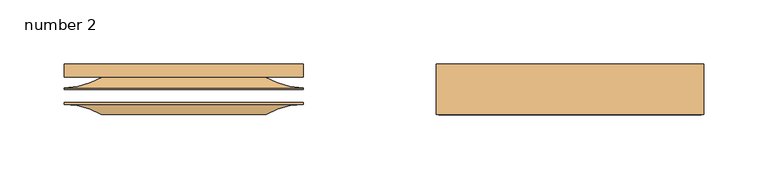
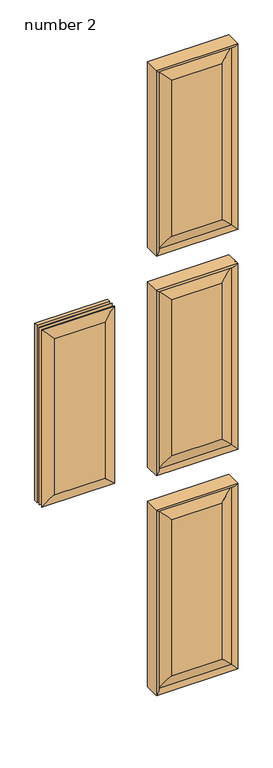
"""IFC4 building model written with IfcOpenShell, lengths in millimetres: door geometry, Door-Interior-Karona-K5660-6_Panel : number 2."""

from ifc_helpers import new_model, si_unit, frame, origin, place, context, project, spatial, polyline, ellipse_curve, source, transform, mapped, element, save
from ifc_brep_helpers import plane_surface, cylinder_surface, revolved_surface, advanced_brep


def number_2_a8c36a05(model_context):
    return source(origin(), model_context, "Body", "AdvancedBrep", [
        advanced_brep(
        [(242.8748, 54.4576, 1893.8748), (242.8748, 54.4576, 1414.4752), (57.1627, 54.4576, 1414.4752), (57.1627, 54.4576, 1893.8748), (242.8748, 34.7218, 1893.8748), (242.8748, 36.0454899, 1893.8748), (57.1627, 36.0454899, 1893.8748), (57.1627, 34.7218, 1893.8748), (57.1627, 44.5515929, 1893.8748), (242.8748, 44.5515929, 1893.8748), (57.1627, 34.7218, 1414.4752), (57.1627, 36.0454899, 1414.4752), (242.8748, 36.0454899, 1414.4752), (242.8748, 34.7218, 1414.4752), (242.8748, 44.5515929, 1414.4752), (57.1627, 44.5515929, 1414.4752), (87.1686653, 44.5515929, 1863.8688347), (212.8688347, 44.5515929, 1863.8688347), (87.1686653, 44.5515929, 1444.4811653), (212.8688347, 44.5515929, 1444.4811653)],
        [
            (0, 1),
            (1, 2),
            (2, 3),
            (3, 0),
            (4, 5),
            (5, 6),
            (6, 7),
            (7, 4),
            (3, 8),
            (8, 9),
            (9, 0),
            (10, 11),
            (11, 12),
            (12, 13),
            (13, 10),
            (1, 14),
            (14, 15),
            (15, 2),
            (9, 14),
            (12, 5),
            (4, 13),
            (6, 11),
            (10, 7),
            (15, 8),
            (16, 6, ellipse_curve(frame((55.2243315, 100.0605261, 1895.8131685), z_axis=(-0.7071067811865475, 0.0, -0.7071067811865475), x_axis=(0.7071067811865476, 0.0, -0.7071067811865474)), 90.5724254, 64.0443762)),
            (5, 17, ellipse_curve(frame((244.8131685, 100.0605261, 1895.8131685), z_axis=(0.7071067811865475, 0.0, -0.7071067811865475), x_axis=(0.7071067811865476, 0.0, 0.7071067811865474)), 90.5724254, 64.0443762)),
            (17, 16),
            (18, 11, ellipse_curve(frame((55.2243315, 100.0605261, 1412.5368315), z_axis=(0.7071067811865475, 0.0, -0.7071067811865475), x_axis=(0.7071067811865474, 0.0, 0.7071067811865476)), 90.5724254, 64.0443762)),
            (16, 18),
            (19, 12, ellipse_curve(frame((244.8131685, 100.0605261, 1412.5368315), z_axis=(0.7071067811865475, 0.0, 0.7071067811865475), x_axis=(-0.7071067811865476, 0.0, 0.7071067811865474)), 90.5724254, 64.0443762)),
            (18, 19),
            (19, 17),
        ],
        [
            plane_surface(frame((57.1627, 54.4576, 1893.8748), z_axis=(0.0, 1.0, 0.0), x_axis=(0.0, 0.0, -1.0))),
            plane_surface(frame((57.1627, 34.7218, 1893.8748), z_axis=(0.0, 0.0, 1.0), x_axis=(-1.0, 0.0, 0.0))),
            plane_surface(frame((57.1627, 34.7218, 1414.4752), z_axis=(0.0, 0.0, -1.0), x_axis=(1.0, 0.0, 0.0))),
            plane_surface(frame((242.8748, 54.4576, 1893.8748), z_axis=(1.0, 0.0, 0.0), x_axis=(0.0, 0.0, -1.0))),
            plane_surface(frame((57.1627, 34.7218, 1893.8748), z_axis=(-1.0, 0.0, 0.0), x_axis=(0.0, 0.0, -1.0))),
            plane_surface(frame((242.8748, 34.7218, 1893.8748), z_axis=(0.0, -1.0, 0.0), x_axis=(0.0, 0.0, -1.0))),
            revolved_surface(polyline([(308.8575446888527, 100.0605261, 1831.7687923), (-8.820044688852704, 100.0605261, 1831.7687923)]), (254.0, 100.0605261, 1895.8131685), (1.0, 0.0, 0.0)),
            revolved_surface(polyline([(119.2687077, 100.0605261, 1959.8575446888528), (119.2687077, 100.0605261, 1348.4924553111473)]), (55.2243315, 100.0605261, 1905.0), (0.0, 0.0, 1.0)),
            revolved_surface(polyline([(-8.820044688852683, 100.0605261, 1476.5812077), (308.8575446888527, 100.0605261, 1476.5812077)]), (46.0375, 100.0605261, 1412.5368315), (-1.0, 0.0, 0.0)),
            revolved_surface(polyline([(180.76879229999997, 100.0605261, 1348.4924553111473), (180.76879229999997, 100.0605261, 1959.8575446888526)]), (244.8131685, 100.0605261, 1403.35), (0.0, 0.0, -1.0)),
            plane_surface(frame((254.0, 44.5515929, 1403.35), z_axis=(0.0, -1.0, 0.0), x_axis=(0.0, 0.0, 1.0))),
        ],
        [
            (0, [[1, 2, 3, 4]]),
            (1, [[5, 6, 7, 8]]),
            (1, [[9, 10, 11, -4]]),
            (2, [[12, 13, 14, 15]]),
            (2, [[16, 17, 18, -2]]),
            (3, [[-11, 19, -16, -1]]),
            (3, [[-14, 20, -5, 21]]),
            (4, [[-7, 22, -12, 23]]),
            (4, [[-18, 24, -9, -3]]),
            (5, [[-23, -15, -21, -8]]),
            (6, [[25, -6, 26, 27]]),
            (7, [[28, -22, -25, 29]]),
            (8, [[30, -13, -28, 31]]),
            (9, [[-26, -20, -30, 32]]),
            (10, [[-24, -17, -19, -10], [-32, -31, -29, -27]]),
        ],
    ),
        advanced_brep(
        [(242.8748, 24.6126, 1893.8748), (242.8748, 24.6126, 1414.4752), (57.1627, 24.6126, 1414.4752), (57.1627, 24.6126, 1893.8748), (214.0448579, 15.4432, 1443.3051421), (214.0448579, 15.4432, 1865.0448579), (85.9926421, 15.4432, 1865.0448579), (85.9926421, 15.4432, 1443.3051421), (57.1627, 23.2889101, 1893.8748), (242.8748, 23.2889101, 1893.8748), (242.8748, 23.2889101, 1414.4752), (57.1627, 23.2889101, 1414.4752)],
        [
            (0, 1),
            (1, 2),
            (2, 3),
            (3, 0),
            (4, 5),
            (5, 6),
            (6, 7),
            (7, 4),
            (3, 8),
            (8, 9),
            (9, 0),
            (1, 10),
            (10, 11),
            (11, 2),
            (7, 11, ellipse_curve(frame((55.2243315, -40.7261261, 1412.5368315), z_axis=(-0.7071067811865475, 0.0, 0.7071067811865475), x_axis=(-0.7071067811865476, 0.0, -0.7071067811865474)), 90.5724254, 64.0443762)),
            (10, 4, ellipse_curve(frame((244.8131685, -40.7261261, 1412.5368315), z_axis=(0.7071067811865475, 0.0, 0.7071067811865475), x_axis=(-0.7071067811865476, 0.0, 0.7071067811865474)), 90.5724254, 64.0443762)),
            (10, 9),
            (9, 5, ellipse_curve(frame((244.8131685, -40.7261261, 1895.8131685), z_axis=(-0.7071067811865475, 0.0, 0.7071067811865475), x_axis=(-0.7071067811865474, 0.0, -0.7071067811865476)), 90.5724254, 64.0443762)),
            (8, 6, ellipse_curve(frame((55.2243315, -40.7261261, 1895.8131685), z_axis=(-0.7071067811865475, 0.0, -0.7071067811865475), x_axis=(0.7071067811865476, 0.0, -0.7071067811865474)), 90.5724254, 64.0443762)),
            (8, 11),
        ],
        [
            plane_surface(frame((57.1627, 24.6126, 1893.8748), z_axis=(0.0, 1.0, 0.0), x_axis=(0.0, 0.0, -1.0))),
            plane_surface(frame((242.8748, 15.4432, 1893.8748), z_axis=(0.0, -1.0, 0.0), x_axis=(0.0, 0.0, -1.0))),
            plane_surface(frame((57.1627, 34.7218, 1893.8748), z_axis=(0.0, 0.0, 1.0), x_axis=(-1.0, 0.0, 0.0))),
            plane_surface(frame((57.1627, 34.7218, 1414.4752), z_axis=(0.0, 0.0, -1.0), x_axis=(1.0, 0.0, 0.0))),
            revolved_surface(polyline([(-8.820044688852711, -40.7261261, 1476.5812077), (308.8575446888527, -40.7261261, 1476.5812077)]), (46.0375, -40.7261261, 1412.5368315), (-1.0, 0.0, 0.0)),
            revolved_surface(polyline([(180.76879229999997, -40.7261261, 1348.4924553111473), (180.76879229999997, -40.7261261, 1959.8575446888528)]), (244.8131685, -40.7261261, 1403.35), (0.0, 0.0, -1.0)),
            revolved_surface(polyline([(308.85754468885267, -40.7261261, 1831.7687923), (-8.820044688852704, -40.7261261, 1831.7687923)]), (254.0, -40.7261261, 1895.8131685), (1.0, 0.0, 0.0)),
            revolved_surface(polyline([(119.2687077, -40.7261261, 1959.8575446888528), (119.2687077, -40.7261261, 1348.4924553111473)]), (55.2243315, -40.7261261, 1905.0), (0.0, 0.0, 1.0)),
            plane_surface(frame((242.8748, 24.6126, 1893.8748), z_axis=(1.0, 0.0, 0.0), x_axis=(0.0, 0.0, -1.0))),
            plane_surface(frame((57.1627, 15.4432, 1893.8748), z_axis=(-1.0, 0.0, 0.0), x_axis=(0.0, 0.0, -1.0))),
        ],
        [
            (0, [[1, 2, 3, 4]]),
            (1, [[5, 6, 7, 8]]),
            (2, [[9, 10, 11, -4]]),
            (3, [[12, 13, 14, -2]]),
            (4, [[-8, 15, -13, 16]]),
            (5, [[17, 18, -5, -16]]),
            (6, [[-10, 19, -6, -18]]),
            (7, [[20, -15, -7, -19]]),
            (8, [[-11, -17, -12, -1]]),
            (9, [[-14, -20, -9, -3]]),
        ],
    ),
        advanced_brep(
        [(254.0, 15.2908, 1905.0), (46.0375, 15.2908, 1905.0), (57.3628137, 24.6126, 1893.6746863), (242.6746863, 24.6126, 1893.6746863), (57.1627, 46.3324899, 1893.8748), (57.1627, 46.3324899, 1414.4752), (48.2727, 54.4576, 1405.5852), (48.2727, 54.4576, 1902.7648), (242.8748, 46.3324899, 1414.4752), (242.8748, 46.3324899, 1893.8748), (251.7648, 54.4576, 1902.7648), (251.7648, 54.4576, 1405.5852), (46.0375, 54.4576, 1403.35), (254.0, 54.4576, 1403.35), (254.0, 15.2908, 1403.35), (46.0375, 15.2908, 1403.35), (57.1627, 34.7218, 1414.4752), (242.8748, 34.7218, 1414.4752), (47.3075, 24.6126, 1903.73), (47.3075, 24.6126, 1404.62), (47.3075, 34.7218, 1404.62), (47.3075, 34.7218, 1903.73), (252.73, 24.6126, 1404.62), (252.73, 24.6126, 1903.73), (57.3628137, 24.6126, 1414.6753137), (242.6746863, 24.6126, 1414.6753137), (252.73, 34.7218, 1404.62), (254.0, 54.4576, 1905.0), (242.8748, 34.7218, 1893.8748), (252.73, 34.7218, 1903.73), (46.0375, 54.4576, 1905.0), (57.1627, 34.7218, 1893.8748)],
        [
            (0, 1),
            (1, 2, ellipse_curve(frame((47.0685124, 25.5788135, 1903.9689876), z_axis=(0.7071067811865475, 0.0, 0.7071067811865475), x_axis=(0.7071067811865476, 0.0, -0.7071067811865474)), 14.6223259, 10.3395458)),
            (2, 3),
            (3, 0, ellipse_curve(frame((252.9689876, 25.5788135, 1903.9689876), z_axis=(-0.7071067811865475, 0.0, 0.7071067811865475), x_axis=(0.7071067811865476, 0.0, 0.7071067811865474)), 14.6223259, 10.3395458)),
            (4, 5),
            (5, 6, ellipse_curve(frame((48.2727, 45.531597, 1405.5852), z_axis=(-0.7071067811865475, 0.0, 0.7071067811865475), x_axis=(0.7071067811865474, 0.0, 0.7071067811865476)), 12.6232745, 8.926003)),
            (6, 7),
            (7, 4, ellipse_curve(frame((48.2727, 45.531597, 1902.7648), z_axis=(-0.7071067811865475, 0.0, -0.7071067811865475), x_axis=(-0.7071067811865474, 0.0, 0.7071067811865476)), 12.6232745, 8.926003)),
            (8, 9),
            (9, 10, ellipse_curve(frame((251.7648, 45.531597, 1902.7648), z_axis=(0.7071067811865475, 0.0, -0.7071067811865475), x_axis=(-0.7071067811865474, 0.0, -0.7071067811865476)), 12.6232745, 8.926003)),
            (10, 11),
            (11, 8, ellipse_curve(frame((251.7648, 45.531597, 1405.5852), z_axis=(0.7071067811865475, 0.0, 0.7071067811865475), x_axis=(0.7071067811865474, 0.0, -0.7071067811865476)), 12.6232745, 8.926003)),
            (12, 13),
            (13, 14),
            (14, 15),
            (15, 12),
            (16, 17),
            (17, 8),
            (8, 5),
            (5, 16),
            (18, 19),
            (19, 20),
            (20, 21),
            (21, 18),
            (22, 19),
            (18, 23),
            (23, 22),
            (24, 25),
            (25, 3),
            (2, 24),
            (22, 26),
            (26, 20),
            (13, 27),
            (27, 0),
            (0, 14),
            (17, 28),
            (28, 9),
            (23, 29),
            (29, 26),
            (27, 30),
            (30, 1),
            (28, 31),
            (31, 4),
            (4, 9),
            (21, 29),
            (30, 12),
            (15, 1),
            (31, 16),
            (6, 11),
            (10, 7),
            (14, 25, ellipse_curve(frame((252.9689876, 25.5788135, 1404.3810124), z_axis=(-0.7071067811865475, 0.0, -0.7071067811865475), x_axis=(-0.7071067811865476, 0.0, 0.7071067811865474)), 14.6223259, 10.3395458)),
            (24, 15, ellipse_curve(frame((47.0685124, 25.5788135, 1404.3810124), z_axis=(0.7071067811865475, 0.0, -0.7071067811865475), x_axis=(-0.7071067811865476, 0.0, -0.7071067811865474)), 14.6223259, 10.3395458)),
        ],
        [
            cylinder_surface(frame((254.0, 25.5788135, 1903.9689876), z_axis=(1.0, 0.0, 0.0), x_axis=(0.0, -1.0, 0.0)), 10.3395458),
            cylinder_surface(frame((48.2727, 45.531597, 1905.0), z_axis=(0.0, 0.0, 1.0), x_axis=(0.0, -1.0, 0.0)), 8.926003),
            cylinder_surface(frame((251.7648, 45.531597, 1403.35), z_axis=(0.0, 0.0, -1.0), x_axis=(0.0, -1.0, 0.0)), 8.926003),
            plane_surface(frame((46.0375, 15.2908, 1403.35), z_axis=(0.0, 0.0, -1.0), x_axis=(1.0, 0.0, 0.0))),
            plane_surface(frame((57.1627, 46.3324899, 1414.4752), z_axis=(0.0, 0.0, 1.0), x_axis=(1.0, 0.0, 0.0))),
            plane_surface(frame((47.3075, 34.7218, 1903.73), z_axis=(1.0, 0.0, 0.0), x_axis=(0.0, 0.0, -1.0))),
            plane_surface(frame((47.3075, 24.6126, 1903.73), z_axis=(0.0, 1.0, 0.0), x_axis=(0.0, 0.0, -1.0))),
            plane_surface(frame((47.3075, 34.7218, 1404.62), z_axis=(0.0, 0.0, 1.0), x_axis=(1.0, 0.0, 0.0))),
            plane_surface(frame((254.0, 15.2908, 1403.35), z_axis=(1.0, 0.0, 0.0), x_axis=(0.0, 0.0, 1.0))),
            plane_surface(frame((242.8748, 46.3324899, 1414.4752), z_axis=(-1.0, 0.0, 0.0), x_axis=(0.0, 0.0, 1.0))),
            plane_surface(frame((252.73, 34.7218, 1404.62), z_axis=(-1.0, 0.0, 0.0), x_axis=(0.0, 0.0, 1.0))),
            plane_surface(frame((254.0, 15.2908, 1905.0), z_axis=(0.0, 0.0, 1.0), x_axis=(-1.0, 0.0, 0.0))),
            plane_surface(frame((242.8748, 46.3324899, 1893.8748), z_axis=(0.0, 0.0, -1.0), x_axis=(-1.0, 0.0, 0.0))),
            plane_surface(frame((252.73, 34.7218, 1903.73), z_axis=(0.0, 0.0, -1.0), x_axis=(-1.0, 0.0, 0.0))),
            plane_surface(frame((46.0375, 15.2908, 1905.0), z_axis=(-1.0, 0.0, 0.0), x_axis=(0.0, 0.0, -1.0))),
            plane_surface(frame((57.1627, 46.3324899, 1893.8748), z_axis=(1.0, 0.0, 0.0), x_axis=(0.0, 0.0, -1.0))),
            plane_surface(frame((57.1627, 34.7218, 1893.8748), z_axis=(0.0, -1.0, 0.0), x_axis=(0.0, 0.0, -1.0))),
            plane_surface(frame((46.0375, 54.4576, 1905.0), z_axis=(0.0, 1.0, 0.0), x_axis=(0.0, 0.0, -1.0))),
            cylinder_surface(frame((46.0375, 45.531597, 1405.5852), z_axis=(-1.0, 0.0, 0.0), x_axis=(0.0, -1.0, 0.0)), 8.926003),
            cylinder_surface(frame((46.0375, 25.5788135, 1404.3810124), z_axis=(-1.0, 0.0, 0.0), x_axis=(0.0, -1.0, 0.0)), 10.3395458),
            cylinder_surface(frame((252.9689876, 25.5788135, 1403.35), z_axis=(0.0, 0.0, -1.0), x_axis=(0.0, -1.0, 0.0)), 10.3395458),
            cylinder_surface(frame((254.0, 45.531597, 1902.7648), z_axis=(1.0, 0.0, 0.0), x_axis=(0.0, -1.0, 0.0)), 8.926003),
            cylinder_surface(frame((47.0685124, 25.5788135, 1905.0), z_axis=(0.0, 0.0, 1.0), x_axis=(0.0, -1.0, 0.0)), 10.3395458),
        ],
        [
            (0, [[1, 2, 3, 4]]),
            (1, [[5, 6, 7, 8]]),
            (2, [[9, 10, 11, 12]]),
            (3, [[13, 14, 15, 16]]),
            (4, [[17, 18, 19, 20]]),
            (5, [[21, 22, 23, 24]]),
            (6, [[25, -21, 26, 27], [28, 29, -3, 30]]),
            (7, [[-25, 31, 32, -22]]),
            (8, [[33, 34, 35, -14]]),
            (9, [[36, 37, -9, -18]]),
            (10, [[-27, 38, 39, -31]]),
            (11, [[40, 41, -1, -34]]),
            (12, [[42, 43, 44, -37]]),
            (13, [[-26, -24, 45, -38]]),
            (14, [[46, -16, 47, -41]]),
            (15, [[48, -20, -5, -43]]),
            (16, [[-32, -39, -45, -23], [-17, -48, -42, -36]]),
            (17, [[-13, -46, -40, -33], [49, -11, 50, -7]]),
            (18, [[-19, -12, -49, -6]]),
            (19, [[-15, 51, -28, 52]]),
            (20, [[-35, -4, -29, -51]]),
            (21, [[-44, -8, -50, -10]]),
            (22, [[-47, -52, -30, -2]]),
        ],
    ),
        advanced_brep(
        [(242.8748, 54.4576, 1300.1498), (242.8748, 54.4576, 820.7502), (57.1627, 54.4576, 820.7502), (57.1627, 54.4576, 1300.1498), (242.8748, 34.7218, 1300.1498), (242.8748, 36.0454899, 1300.1498), (57.1627, 36.0454899, 1300.1498), (57.1627, 34.7218, 1300.1498), (57.1627, 44.5515929, 1300.1498), (242.8748, 44.5515929, 1300.1498), (57.1627, 34.7218, 820.7502), (57.1627, 36.0454899, 820.7502), (242.8748, 36.0454899, 820.7502), (242.8748, 34.7218, 820.7502), (242.8748, 44.5515929, 820.7502), (57.1627, 44.5515929, 820.7502), (87.1686653, 44.5515929, 1270.1438347), (212.8688347, 44.5515929, 1270.1438347), (87.1686653, 44.5515929, 850.7561653), (212.8688347, 44.5515929, 850.7561653)],
        [
            (0, 1),
            (1, 2),
            (2, 3),
            (3, 0),
            (4, 5),
            (5, 6),
            (6, 7),
            (7, 4),
            (3, 8),
            (8, 9),
            (9, 0),
            (10, 11),
            (11, 12),
            (12, 13),
            (13, 10),
            (1, 14),
            (14, 15),
            (15, 2),
            (9, 14),
            (12, 5),
            (4, 13),
            (6, 11),
            (10, 7),
            (15, 8),
            (16, 6, ellipse_curve(frame((55.2243315, 100.0605261, 1302.0881685), z_axis=(-0.7071067811865475, 0.0, -0.7071067811865475), x_axis=(0.7071067811865476, 0.0, -0.7071067811865474)), 90.5724254, 64.0443762)),
            (5, 17, ellipse_curve(frame((244.8131685, 100.0605261, 1302.0881685), z_axis=(0.7071067811865475, 0.0, -0.7071067811865475), x_axis=(0.7071067811865476, 0.0, 0.7071067811865474)), 90.5724254, 64.0443762)),
            (17, 16),
            (18, 11, ellipse_curve(frame((55.2243315, 100.0605261, 818.8118315), z_axis=(0.7071067811865475, 0.0, -0.7071067811865475), x_axis=(0.7071067811865474, 0.0, 0.7071067811865476)), 90.5724254, 64.0443762)),
            (16, 18),
            (19, 12, ellipse_curve(frame((244.8131685, 100.0605261, 818.8118315), z_axis=(0.7071067811865475, 0.0, 0.7071067811865475), x_axis=(-0.7071067811865476, 0.0, 0.7071067811865474)), 90.5724254, 64.0443762)),
            (18, 19),
            (19, 17),
        ],
        [
            plane_surface(frame((57.1627, 54.4576, 1300.1498), z_axis=(0.0, 1.0, 0.0), x_axis=(0.0, 0.0, -1.0))),
            plane_surface(frame((57.1627, 34.7218, 1300.1498), z_axis=(0.0, 0.0, 1.0), x_axis=(-1.0, 0.0, 0.0))),
            plane_surface(frame((57.1627, 34.7218, 820.7502), z_axis=(0.0, 0.0, -1.0), x_axis=(1.0, 0.0, 0.0))),
            plane_surface(frame((242.8748, 54.4576, 1300.1498), z_axis=(1.0, 0.0, 0.0), x_axis=(0.0, 0.0, -1.0))),
            plane_surface(frame((57.1627, 34.7218, 1300.1498), z_axis=(-1.0, 0.0, 0.0), x_axis=(0.0, 0.0, -1.0))),
            plane_surface(frame((242.8748, 34.7218, 1300.1498), z_axis=(0.0, -1.0, 0.0), x_axis=(0.0, 0.0, -1.0))),
            revolved_surface(polyline([(308.8575446888527, 100.0605261, 1238.0437923), (-8.820044688852704, 100.0605261, 1238.0437923)]), (254.0, 100.0605261, 1302.0881685), (1.0, 0.0, 0.0)),
            revolved_surface(polyline([(119.2687077, 100.0605261, 1366.1325446888527), (119.2687077, 100.0605261, 754.7674553111474)]), (55.2243315, 100.0605261, 1311.275), (0.0, 0.0, 1.0)),
            revolved_surface(polyline([(-8.820044688852683, 100.0605261, 882.8562077), (308.8575446888527, 100.0605261, 882.8562077)]), (46.0375, 100.0605261, 818.8118315), (-1.0, 0.0, 0.0)),
            revolved_surface(polyline([(180.76879229999997, 100.0605261, 754.7674553111474), (180.76879229999997, 100.0605261, 1366.1325446888527)]), (244.8131685, 100.0605261, 809.625), (0.0, 0.0, -1.0)),
            plane_surface(frame((254.0, 44.5515929, 809.625), z_axis=(0.0, -1.0, 0.0), x_axis=(0.0, 0.0, 1.0))),
        ],
        [
            (0, [[1, 2, 3, 4]]),
            (1, [[5, 6, 7, 8]]),
            (1, [[9, 10, 11, -4]]),
            (2, [[12, 13, 14, 15]]),
            (2, [[16, 17, 18, -2]]),
            (3, [[-11, 19, -16, -1]]),
            (3, [[-14, 20, -5, 21]]),
            (4, [[-7, 22, -12, 23]]),
            (4, [[-18, 24, -9, -3]]),
            (5, [[-23, -15, -21, -8]]),
            (6, [[25, -6, 26, 27]]),
            (7, [[28, -22, -25, 29]]),
            (8, [[30, -13, -28, 31]]),
            (9, [[-26, -20, -30, 32]]),
            (10, [[-24, -17, -19, -10], [-32, -31, -29, -27]]),
        ],
    ),
        advanced_brep(
        [(242.8748, 24.6126, 1300.1498), (242.8748, 24.6126, 820.7502), (57.1627, 24.6126, 820.7502), (57.1627, 24.6126, 1300.1498), (214.0448579, 15.4432, 849.5801421), (214.0448579, 15.4432, 1271.3198579), (85.9926421, 15.4432, 1271.3198579), (85.9926421, 15.4432, 849.5801421), (57.1627, 23.2889101, 1300.1498), (242.8748, 23.2889101, 1300.1498), (242.8748, 23.2889101, 820.7502), (57.1627, 23.2889101, 820.7502)],
        [
            (0, 1),
            (1, 2),
            (2, 3),
            (3, 0),
            (4, 5),
            (5, 6),
            (6, 7),
            (7, 4),
            (3, 8),
            (8, 9),
            (9, 0),
            (1, 10),
            (10, 11),
            (11, 2),
            (7, 11, ellipse_curve(frame((55.2243315, -40.7261261, 818.8118315), z_axis=(-0.7071067811865475, 0.0, 0.7071067811865475), x_axis=(-0.7071067811865476, 0.0, -0.7071067811865474)), 90.5724254, 64.0443762)),
            (10, 4, ellipse_curve(frame((244.8131685, -40.7261261, 818.8118315), z_axis=(0.7071067811865475, 0.0, 0.7071067811865475), x_axis=(-0.7071067811865476, 0.0, 0.7071067811865474)), 90.5724254, 64.0443762)),
            (10, 9),
            (9, 5, ellipse_curve(frame((244.8131685, -40.7261261, 1302.0881685), z_axis=(-0.7071067811865475, 0.0, 0.7071067811865475), x_axis=(-0.7071067811865474, 0.0, -0.7071067811865476)), 90.5724254, 64.0443762)),
            (8, 6, ellipse_curve(frame((55.2243315, -40.7261261, 1302.0881685), z_axis=(-0.7071067811865475, 0.0, -0.7071067811865475), x_axis=(0.7071067811865476, 0.0, -0.7071067811865474)), 90.5724254, 64.0443762)),
            (8, 11),
        ],
        [
            plane_surface(frame((57.1627, 24.6126, 1300.1498), z_axis=(0.0, 1.0, 0.0), x_axis=(0.0, 0.0, -1.0))),
            plane_surface(frame((242.8748, 15.4432, 1300.1498), z_axis=(0.0, -1.0, 0.0), x_axis=(0.0, 0.0, -1.0))),
            plane_surface(frame((57.1627, 34.7218, 1300.1498), z_axis=(0.0, 0.0, 1.0), x_axis=(-1.0, 0.0, 0.0))),
            plane_surface(frame((57.1627, 34.7218, 820.7502), z_axis=(0.0, 0.0, -1.0), x_axis=(1.0, 0.0, 0.0))),
            revolved_surface(polyline([(-8.820044688852711, -40.7261261, 882.8562077), (308.8575446888527, -40.7261261, 882.8562077)]), (46.0375, -40.7261261, 818.8118315), (-1.0, 0.0, 0.0)),
            revolved_surface(polyline([(180.76879229999997, -40.7261261, 754.7674553111474), (180.76879229999997, -40.7261261, 1366.1325446888527)]), (244.8131685, -40.7261261, 809.625), (0.0, 0.0, -1.0)),
            revolved_surface(polyline([(308.85754468885267, -40.7261261, 1238.0437923), (-8.820044688852704, -40.7261261, 1238.0437923)]), (254.0, -40.7261261, 1302.0881685), (1.0, 0.0, 0.0)),
            revolved_surface(polyline([(119.2687077, -40.7261261, 1366.1325446888527), (119.2687077, -40.7261261, 754.7674553111474)]), (55.2243315, -40.7261261, 1311.275), (0.0, 0.0, 1.0)),
            plane_surface(frame((242.8748, 24.6126, 1300.1498), z_axis=(1.0, 0.0, 0.0), x_axis=(0.0, 0.0, -1.0))),
            plane_surface(frame((57.1627, 15.4432, 1300.1498), z_axis=(-1.0, 0.0, 0.0), x_axis=(0.0, 0.0, -1.0))),
        ],
        [
            (0, [[1, 2, 3, 4]]),
            (1, [[5, 6, 7, 8]]),
            (2, [[9, 10, 11, -4]]),
            (3, [[12, 13, 14, -2]]),
            (4, [[-8, 15, -13, 16]]),
            (5, [[17, 18, -5, -16]]),
            (6, [[-10, 19, -6, -18]]),
            (7, [[20, -15, -7, -19]]),
            (8, [[-11, -17, -12, -1]]),
            (9, [[-14, -20, -9, -3]]),
        ],
    ),
        advanced_brep(
        [(254.0, 15.2908, 1311.275), (46.0375, 15.2908, 1311.275), (57.3628137, 24.6126, 1299.9496863), (242.6746863, 24.6126, 1299.9496863), (57.1627, 46.3324899, 1300.1498), (57.1627, 46.3324899, 820.7502), (48.2727, 54.4576, 811.8602), (48.2727, 54.4576, 1309.0398), (242.8748, 46.3324899, 820.7502), (242.8748, 46.3324899, 1300.1498), (251.7648, 54.4576, 1309.0398), (251.7648, 54.4576, 811.8602), (46.0375, 54.4576, 809.625), (254.0, 54.4576, 809.625), (254.0, 15.2908, 809.625), (46.0375, 15.2908, 809.625), (57.1627, 34.7218, 820.7502), (242.8748, 34.7218, 820.7502), (47.3075, 24.6126, 1310.005), (47.3075, 24.6126, 810.895), (47.3075, 34.7218, 810.895), (47.3075, 34.7218, 1310.005), (252.73, 24.6126, 810.895), (252.73, 24.6126, 1310.005), (57.3628137, 24.6126, 820.9503137), (242.6746863, 24.6126, 820.9503137), (252.73, 34.7218, 810.895), (254.0, 54.4576, 1311.275), (242.8748, 34.7218, 1300.1498), (252.73, 34.7218, 1310.005), (46.0375, 54.4576, 1311.275), (57.1627, 34.7218, 1300.1498)],
        [
            (0, 1),
            (1, 2, ellipse_curve(frame((47.0685124, 25.5788135, 1310.2439876), z_axis=(0.7071067811865475, 0.0, 0.7071067811865475), x_axis=(0.7071067811865476, 0.0, -0.7071067811865474)), 14.6223259, 10.3395458)),
            (2, 3),
            (3, 0, ellipse_curve(frame((252.9689876, 25.5788135, 1310.2439876), z_axis=(-0.7071067811865475, 0.0, 0.7071067811865475), x_axis=(0.7071067811865476, 0.0, 0.7071067811865474)), 14.6223259, 10.3395458)),
            (4, 5),
            (5, 6, ellipse_curve(frame((48.2727, 45.531597, 811.8602), z_axis=(-0.7071067811865475, 0.0, 0.7071067811865475), x_axis=(0.7071067811865474, 0.0, 0.7071067811865476)), 12.6232745, 8.926003)),
            (6, 7),
            (7, 4, ellipse_curve(frame((48.2727, 45.531597, 1309.0398), z_axis=(-0.7071067811865475, 0.0, -0.7071067811865475), x_axis=(-0.7071067811865474, 0.0, 0.7071067811865476)), 12.6232745, 8.926003)),
            (8, 9),
            (9, 10, ellipse_curve(frame((251.7648, 45.531597, 1309.0398), z_axis=(0.7071067811865475, 0.0, -0.7071067811865475), x_axis=(-0.7071067811865474, 0.0, -0.7071067811865476)), 12.6232745, 8.926003)),
            (10, 11),
            (11, 8, ellipse_curve(frame((251.7648, 45.531597, 811.8602), z_axis=(0.7071067811865475, 0.0, 0.7071067811865475), x_axis=(0.7071067811865474, 0.0, -0.7071067811865476)), 12.6232745, 8.926003)),
            (12, 13),
            (13, 14),
            (14, 15),
            (15, 12),
            (16, 17),
            (17, 8),
            (8, 5),
            (5, 16),
            (18, 19),
            (19, 20),
            (20, 21),
            (21, 18),
            (22, 19),
            (18, 23),
            (23, 22),
            (24, 25),
            (25, 3),
            (2, 24),
            (14, 25, ellipse_curve(frame((252.9689876, 25.5788135, 810.6560124), z_axis=(-0.7071067811865475, 0.0, -0.7071067811865475), x_axis=(-0.7071067811865476, 0.0, 0.7071067811865474)), 14.6223259, 10.3395458)),
            (24, 15, ellipse_curve(frame((47.0685124, 25.5788135, 810.6560124), z_axis=(0.7071067811865475, 0.0, -0.7071067811865475), x_axis=(-0.7071067811865476, 0.0, -0.7071067811865474)), 14.6223259, 10.3395458)),
            (22, 26),
            (26, 20),
            (13, 27),
            (27, 0),
            (0, 14),
            (17, 28),
            (28, 9),
            (23, 29),
            (29, 26),
            (27, 30),
            (30, 1),
            (28, 31),
            (31, 4),
            (4, 9),
            (21, 29),
            (30, 12),
            (15, 1),
            (31, 16),
            (6, 11),
            (10, 7),
        ],
        [
            cylinder_surface(frame((254.0, 25.5788135, 1310.2439876), z_axis=(1.0, 0.0, 0.0), x_axis=(0.0, -1.0, 0.0)), 10.3395458),
            cylinder_surface(frame((48.2727, 45.531597, 1311.275), z_axis=(0.0, 0.0, 1.0), x_axis=(0.0, -1.0, 0.0)), 8.926003),
            cylinder_surface(frame((251.7648, 45.531597, 809.625), z_axis=(0.0, 0.0, -1.0), x_axis=(0.0, -1.0, 0.0)), 8.926003),
            plane_surface(frame((46.0375, 15.2908, 809.625), z_axis=(0.0, 0.0, -1.0), x_axis=(1.0, 0.0, 0.0))),
            plane_surface(frame((57.1627, 46.3324899, 820.7502), z_axis=(0.0, 0.0, 1.0), x_axis=(1.0, 0.0, 0.0))),
            plane_surface(frame((47.3075, 34.7218, 1310.005), z_axis=(1.0, 0.0, 0.0), x_axis=(0.0, 0.0, -1.0))),
            plane_surface(frame((47.3075, 24.6126, 1310.005), z_axis=(0.0, 1.0, 0.0), x_axis=(0.0, 0.0, -1.0))),
            cylinder_surface(frame((46.0375, 25.5788135, 810.6560124), z_axis=(-1.0, 0.0, 0.0), x_axis=(0.0, -1.0, 0.0)), 10.3395458),
            plane_surface(frame((47.3075, 34.7218, 810.895), z_axis=(0.0, 0.0, 1.0), x_axis=(1.0, 0.0, 0.0))),
            plane_surface(frame((254.0, 15.2908, 809.625), z_axis=(1.0, 0.0, 0.0), x_axis=(0.0, 0.0, 1.0))),
            plane_surface(frame((242.8748, 46.3324899, 820.7502), z_axis=(-1.0, 0.0, 0.0), x_axis=(0.0, 0.0, 1.0))),
            plane_surface(frame((252.73, 34.7218, 810.895), z_axis=(-1.0, 0.0, 0.0), x_axis=(0.0, 0.0, 1.0))),
            plane_surface(frame((254.0, 15.2908, 1311.275), z_axis=(0.0, 0.0, 1.0), x_axis=(-1.0, 0.0, 0.0))),
            plane_surface(frame((242.8748, 46.3324899, 1300.1498), z_axis=(0.0, 0.0, -1.0), x_axis=(-1.0, 0.0, 0.0))),
            plane_surface(frame((252.73, 34.7218, 1310.005), z_axis=(0.0, 0.0, -1.0), x_axis=(-1.0, 0.0, 0.0))),
            plane_surface(frame((46.0375, 15.2908, 1311.275), z_axis=(-1.0, 0.0, 0.0), x_axis=(0.0, 0.0, -1.0))),
            plane_surface(frame((57.1627, 46.3324899, 1300.1498), z_axis=(1.0, 0.0, 0.0), x_axis=(0.0, 0.0, -1.0))),
            plane_surface(frame((57.1627, 34.7218, 1300.1498), z_axis=(0.0, -1.0, 0.0), x_axis=(0.0, 0.0, -1.0))),
            plane_surface(frame((46.0375, 54.4576, 1311.275), z_axis=(0.0, 1.0, 0.0), x_axis=(0.0, 0.0, -1.0))),
            cylinder_surface(frame((46.0375, 45.531597, 811.8602), z_axis=(-1.0, 0.0, 0.0), x_axis=(0.0, -1.0, 0.0)), 8.926003),
            cylinder_surface(frame((252.9689876, 25.5788135, 809.625), z_axis=(0.0, 0.0, -1.0), x_axis=(0.0, -1.0, 0.0)), 10.3395458),
            cylinder_surface(frame((254.0, 45.531597, 1309.0398), z_axis=(1.0, 0.0, 0.0), x_axis=(0.0, -1.0, 0.0)), 8.926003),
            cylinder_surface(frame((47.0685124, 25.5788135, 1311.275), z_axis=(0.0, 0.0, 1.0), x_axis=(0.0, -1.0, 0.0)), 10.3395458),
        ],
        [
            (0, [[1, 2, 3, 4]]),
            (1, [[5, 6, 7, 8]]),
            (2, [[9, 10, 11, 12]]),
            (3, [[13, 14, 15, 16]]),
            (4, [[17, 18, 19, 20]]),
            (5, [[21, 22, 23, 24]]),
            (6, [[25, -21, 26, 27], [28, 29, -3, 30]]),
            (7, [[-15, 31, -28, 32]]),
            (8, [[-25, 33, 34, -22]]),
            (9, [[35, 36, 37, -14]]),
            (10, [[38, 39, -9, -18]]),
            (11, [[-27, 40, 41, -33]]),
            (12, [[42, 43, -1, -36]]),
            (13, [[44, 45, 46, -39]]),
            (14, [[-26, -24, 47, -40]]),
            (15, [[48, -16, 49, -43]]),
            (16, [[50, -20, -5, -45]]),
            (17, [[-34, -41, -47, -23], [-17, -50, -44, -38]]),
            (18, [[-13, -48, -42, -35], [51, -11, 52, -7]]),
            (19, [[-19, -12, -51, -6]]),
            (20, [[-37, -4, -29, -31]]),
            (21, [[-46, -8, -52, -10]]),
            (22, [[-49, -32, -30, -2]]),
        ],
    ),
        advanced_brep(
        [(242.8748, 54.4576, 706.4248), (242.8748, 54.4576, 227.0252), (57.1627, 54.4576, 227.0252), (57.1627, 54.4576, 706.4248), (242.8748, 34.7218, 706.4248), (242.8748, 36.0454899, 706.4248), (57.1627, 36.0454899, 706.4248), (57.1627, 34.7218, 706.4248), (57.1627, 44.5515929, 706.4248), (242.8748, 44.5515929, 706.4248), (57.1627, 34.7218, 227.0252), (57.1627, 36.0454899, 227.0252), (242.8748, 36.0454899, 227.0252), (242.8748, 34.7218, 227.0252), (242.8748, 44.5515929, 227.0252), (57.1627, 44.5515929, 227.0252), (87.1686653, 44.5515929, 676.4188347), (212.8688347, 44.5515929, 676.4188347), (87.1686653, 44.5515929, 257.0311653), (212.8688347, 44.5515929, 257.0311653)],
        [
            (0, 1),
            (1, 2),
            (2, 3),
            (3, 0),
            (4, 5),
            (5, 6),
            (6, 7),
            (7, 4),
            (3, 8),
            (8, 9),
            (9, 0),
            (10, 11),
            (11, 12),
            (12, 13),
            (13, 10),
            (1, 14),
            (14, 15),
            (15, 2),
            (9, 14),
            (12, 5),
            (4, 13),
            (6, 11),
            (10, 7),
            (15, 8),
            (16, 6, ellipse_curve(frame((55.2243315, 100.0605261, 708.3631685), z_axis=(-0.7071067811865475, 0.0, -0.7071067811865475), x_axis=(0.7071067811865476, 0.0, -0.7071067811865474)), 90.5724254, 64.0443762)),
            (5, 17, ellipse_curve(frame((244.8131685, 100.0605261, 708.3631685), z_axis=(0.7071067811865475, 0.0, -0.7071067811865475), x_axis=(0.7071067811865476, 0.0, 0.7071067811865474)), 90.5724254, 64.0443762)),
            (17, 16),
            (18, 11, ellipse_curve(frame((55.2243315, 100.0605261, 225.0868315), z_axis=(0.7071067811865475, 0.0, -0.7071067811865475), x_axis=(0.7071067811865474, 0.0, 0.7071067811865476)), 90.5724254, 64.0443762)),
            (16, 18),
            (19, 12, ellipse_curve(frame((244.8131685, 100.0605261, 225.0868315), z_axis=(0.7071067811865475, 0.0, 0.7071067811865475), x_axis=(-0.7071067811865476, 0.0, 0.7071067811865474)), 90.5724254, 64.0443762)),
            (18, 19),
            (19, 17),
        ],
        [
            plane_surface(frame((57.1627, 54.4576, 706.4248), z_axis=(0.0, 1.0, 0.0), x_axis=(0.0, 0.0, -1.0))),
            plane_surface(frame((57.1627, 34.7218, 706.4248), z_axis=(0.0, 0.0, 1.0), x_axis=(-1.0, 0.0, 0.0))),
            plane_surface(frame((57.1627, 34.7218, 227.0252), z_axis=(0.0, 0.0, -1.0), x_axis=(1.0, 0.0, 0.0))),
            plane_surface(frame((242.8748, 54.4576, 706.4248), z_axis=(1.0, 0.0, 0.0), x_axis=(0.0, 0.0, -1.0))),
            plane_surface(frame((57.1627, 34.7218, 706.4248), z_axis=(-1.0, 0.0, 0.0), x_axis=(0.0, 0.0, -1.0))),
            plane_surface(frame((242.8748, 34.7218, 706.4248), z_axis=(0.0, -1.0, 0.0), x_axis=(0.0, 0.0, -1.0))),
            revolved_surface(polyline([(308.8575446888527, 100.0605261, 644.3187923), (-8.820044688852704, 100.0605261, 644.3187923)]), (254.0, 100.0605261, 708.3631685), (1.0, 0.0, 0.0)),
            revolved_surface(polyline([(119.2687077, 100.0605261, 772.4075446888527), (119.2687077, 100.0605261, 161.04245531114725)]), (55.2243315, 100.0605261, 717.55), (0.0, 0.0, 1.0)),
            revolved_surface(polyline([(-8.820044688852683, 100.0605261, 289.1312077), (308.8575446888527, 100.0605261, 289.1312077)]), (46.0375, 100.0605261, 225.0868315), (-1.0, 0.0, 0.0)),
            revolved_surface(polyline([(180.76879229999997, 100.0605261, 161.0424553111473), (180.76879229999997, 100.0605261, 772.4075446888527)]), (244.8131685, 100.0605261, 215.9), (0.0, 0.0, -1.0)),
            plane_surface(frame((254.0, 44.5515929, 215.9), z_axis=(0.0, -1.0, 0.0), x_axis=(0.0, 0.0, 1.0))),
        ],
        [
            (0, [[1, 2, 3, 4]]),
            (1, [[5, 6, 7, 8]]),
            (1, [[9, 10, 11, -4]]),
            (2, [[12, 13, 14, 15]]),
            (2, [[16, 17, 18, -2]]),
            (3, [[-11, 19, -16, -1]]),
            (3, [[-14, 20, -5, 21]]),
            (4, [[-7, 22, -12, 23]]),
            (4, [[-18, 24, -9, -3]]),
            (5, [[-23, -15, -21, -8]]),
            (6, [[25, -6, 26, 27]]),
            (7, [[28, -22, -25, 29]]),
            (8, [[30, -13, -28, 31]]),
            (9, [[-26, -20, -30, 32]]),
            (10, [[-24, -17, -19, -10], [-32, -31, -29, -27]]),
        ],
    ),
        advanced_brep(
        [(242.8748, 24.6126, 706.4248), (242.8748, 24.6126, 227.0252), (57.1627, 24.6126, 227.0252), (57.1627, 24.6126, 706.4248), (214.0448579, 15.4432, 255.8551421), (214.0448579, 15.4432, 677.5948579), (85.9926421, 15.4432, 677.5948579), (85.9926421, 15.4432, 255.8551421), (57.1627, 23.2889101, 706.4248), (242.8748, 23.2889101, 706.4248), (242.8748, 23.2889101, 227.0252), (57.1627, 23.2889101, 227.0252)],
        [
            (0, 1),
            (1, 2),
            (2, 3),
            (3, 0),
            (4, 5),
            (5, 6),
            (6, 7),
            (7, 4),
            (3, 8),
            (8, 9),
            (9, 0),
            (1, 10),
            (10, 11),
            (11, 2),
            (7, 11, ellipse_curve(frame((55.2243315, -40.7261261, 225.0868315), z_axis=(-0.7071067811865475, 0.0, 0.7071067811865475), x_axis=(-0.7071067811865476, 0.0, -0.7071067811865474)), 90.5724254, 64.0443762)),
            (10, 4, ellipse_curve(frame((244.8131685, -40.7261261, 225.0868315), z_axis=(0.7071067811865475, 0.0, 0.7071067811865475), x_axis=(-0.7071067811865476, 0.0, 0.7071067811865474)), 90.5724254, 64.0443762)),
            (10, 9),
            (9, 5, ellipse_curve(frame((244.8131685, -40.7261261, 708.3631685), z_axis=(-0.7071067811865475, 0.0, 0.7071067811865475), x_axis=(-0.7071067811865474, 0.0, -0.7071067811865476)), 90.5724254, 64.0443762)),
            (8, 6, ellipse_curve(frame((55.2243315, -40.7261261, 708.3631685), z_axis=(-0.7071067811865475, 0.0, -0.7071067811865475), x_axis=(0.7071067811865476, 0.0, -0.7071067811865474)), 90.5724254, 64.0443762)),
            (8, 11),
        ],
        [
            plane_surface(frame((57.1627, 24.6126, 706.4248), z_axis=(0.0, 1.0, 0.0), x_axis=(0.0, 0.0, -1.0))),
            plane_surface(frame((242.8748, 15.4432, 706.4248), z_axis=(0.0, -1.0, 0.0), x_axis=(0.0, 0.0, -1.0))),
            plane_surface(frame((57.1627, 34.7218, 706.4248), z_axis=(0.0, 0.0, 1.0), x_axis=(-1.0, 0.0, 0.0))),
            plane_surface(frame((57.1627, 34.7218, 227.0252), z_axis=(0.0, 0.0, -1.0), x_axis=(1.0, 0.0, 0.0))),
            revolved_surface(polyline([(-8.820044688852711, -40.7261261, 289.1312077), (308.8575446888527, -40.7261261, 289.1312077)]), (46.0375, -40.7261261, 225.0868315), (-1.0, 0.0, 0.0)),
            revolved_surface(polyline([(180.76879229999997, -40.7261261, 161.0424553111473), (180.76879229999997, -40.7261261, 772.4075446888527)]), (244.8131685, -40.7261261, 215.9), (0.0, 0.0, -1.0)),
            revolved_surface(polyline([(308.85754468885267, -40.7261261, 644.3187923), (-8.820044688852704, -40.7261261, 644.3187923)]), (254.0, -40.7261261, 708.3631685), (1.0, 0.0, 0.0)),
            revolved_surface(polyline([(119.2687077, -40.7261261, 772.4075446888527), (119.2687077, -40.7261261, 161.04245531114736)]), (55.2243315, -40.7261261, 717.55), (0.0, 0.0, 1.0)),
            plane_surface(frame((242.8748, 24.6126, 706.4248), z_axis=(1.0, 0.0, 0.0), x_axis=(0.0, 0.0, -1.0))),
            plane_surface(frame((57.1627, 15.4432, 706.4248), z_axis=(-1.0, 0.0, 0.0), x_axis=(0.0, 0.0, -1.0))),
        ],
        [
            (0, [[1, 2, 3, 4]]),
            (1, [[5, 6, 7, 8]]),
            (2, [[9, 10, 11, -4]]),
            (3, [[12, 13, 14, -2]]),
            (4, [[-8, 15, -13, 16]]),
            (5, [[17, 18, -5, -16]]),
            (6, [[-10, 19, -6, -18]]),
            (7, [[20, -15, -7, -19]]),
            (8, [[-11, -17, -12, -1]]),
            (9, [[-14, -20, -9, -3]]),
        ],
    ),
        advanced_brep(
        [(254.0, 15.2908, 717.55), (46.0375, 15.2908, 717.55), (57.3628137, 24.6126, 706.2246863), (242.6746863, 24.6126, 706.2246863), (57.1627, 46.3324899, 706.4248), (57.1627, 46.3324899, 227.0252), (48.2727, 54.4576, 218.1352), (48.2727, 54.4576, 715.3148), (242.8748, 46.3324899, 227.0252), (242.8748, 46.3324899, 706.4248), (251.7648, 54.4576, 715.3148), (251.7648, 54.4576, 218.1352), (46.0375, 54.4576, 215.9), (254.0, 54.4576, 215.9), (254.0, 15.2908, 215.9), (46.0375, 15.2908, 215.9), (57.1627, 34.7218, 227.0252), (242.8748, 34.7218, 227.0252), (47.3075, 24.6126, 716.28), (47.3075, 24.6126, 217.17), (47.3075, 34.7218, 217.17), (47.3075, 34.7218, 716.28), (252.73, 24.6126, 217.17), (252.73, 24.6126, 716.28), (57.3628137, 24.6126, 227.2253137), (242.6746863, 24.6126, 227.2253137), (252.73, 34.7218, 217.17), (254.0, 54.4576, 717.55), (242.8748, 34.7218, 706.4248), (252.73, 34.7218, 716.28), (46.0375, 54.4576, 717.55), (57.1627, 34.7218, 706.4248)],
        [
            (0, 1),
            (1, 2, ellipse_curve(frame((47.0685124, 25.5788135, 716.5189876), z_axis=(0.7071067811865475, 0.0, 0.7071067811865475), x_axis=(0.7071067811865476, 0.0, -0.7071067811865474)), 14.6223259, 10.3395458)),
            (2, 3),
            (3, 0, ellipse_curve(frame((252.9689876, 25.5788135, 716.5189876), z_axis=(-0.7071067811865475, 0.0, 0.7071067811865475), x_axis=(0.7071067811865476, 0.0, 0.7071067811865474)), 14.6223259, 10.3395458)),
            (4, 5),
            (5, 6, ellipse_curve(frame((48.2727, 45.531597, 218.1352), z_axis=(-0.7071067811865475, 0.0, 0.7071067811865475), x_axis=(0.7071067811865474, 0.0, 0.7071067811865476)), 12.6232745, 8.926003)),
            (6, 7),
            (7, 4, ellipse_curve(frame((48.2727, 45.531597, 715.3148), z_axis=(-0.7071067811865475, 0.0, -0.7071067811865475), x_axis=(-0.7071067811865474, 0.0, 0.7071067811865476)), 12.6232745, 8.926003)),
            (8, 9),
            (9, 10, ellipse_curve(frame((251.7648, 45.531597, 715.3148), z_axis=(0.7071067811865475, 0.0, -0.7071067811865475), x_axis=(-0.7071067811865474, 0.0, -0.7071067811865476)), 12.6232745, 8.926003)),
            (10, 11),
            (11, 8, ellipse_curve(frame((251.7648, 45.531597, 218.1352), z_axis=(0.7071067811865475, 0.0, 0.7071067811865475), x_axis=(0.7071067811865474, 0.0, -0.7071067811865476)), 12.6232745, 8.926003)),
            (12, 13),
            (13, 14),
            (14, 15),
            (15, 12),
            (16, 17),
            (17, 8),
            (8, 5),
            (5, 16),
            (18, 19),
            (19, 20),
            (20, 21),
            (21, 18),
            (22, 19),
            (18, 23),
            (23, 22),
            (24, 25),
            (25, 3),
            (2, 24),
            (14, 25, ellipse_curve(frame((252.9689876, 25.5788135, 216.9310124), z_axis=(-0.7071067811865475, 0.0, -0.7071067811865475), x_axis=(-0.7071067811865476, 0.0, 0.7071067811865474)), 14.6223259, 10.3395458)),
            (24, 15, ellipse_curve(frame((47.0685124, 25.5788135, 216.9310124), z_axis=(0.7071067811865475, 0.0, -0.7071067811865475), x_axis=(-0.7071067811865476, 0.0, -0.7071067811865474)), 14.6223259, 10.3395458)),
            (22, 26),
            (26, 20),
            (13, 27),
            (27, 0),
            (0, 14),
            (17, 28),
            (28, 9),
            (23, 29),
            (29, 26),
            (27, 30),
            (30, 1),
            (28, 31),
            (31, 4),
            (4, 9),
            (21, 29),
            (30, 12),
            (15, 1),
            (31, 16),
            (6, 11),
            (10, 7),
        ],
        [
            cylinder_surface(frame((254.0, 25.5788135, 716.5189876), z_axis=(1.0, 0.0, 0.0), x_axis=(0.0, -1.0, 0.0)), 10.3395458),
            cylinder_surface(frame((48.2727, 45.531597, 717.55), z_axis=(0.0, 0.0, 1.0), x_axis=(0.0, -1.0, 0.0)), 8.926003),
            cylinder_surface(frame((251.7648, 45.531597, 215.9), z_axis=(0.0, 0.0, -1.0), x_axis=(0.0, -1.0, 0.0)), 8.926003),
            plane_surface(frame((46.0375, 15.2908, 215.9), z_axis=(0.0, 0.0, -1.0), x_axis=(1.0, 0.0, 0.0))),
            plane_surface(frame((57.1627, 46.3324899, 227.0252), z_axis=(0.0, 0.0, 1.0), x_axis=(1.0, 0.0, 0.0))),
            plane_surface(frame((47.3075, 34.7218, 716.28), z_axis=(1.0, 0.0, 0.0), x_axis=(0.0, 0.0, -1.0))),
            plane_surface(frame((47.3075, 24.6126, 716.28), z_axis=(0.0, 1.0, 0.0), x_axis=(0.0, 0.0, -1.0))),
            cylinder_surface(frame((46.0375, 25.5788135, 216.9310124), z_axis=(-1.0, 0.0, 0.0), x_axis=(0.0, -1.0, 0.0)), 10.3395458),
            plane_surface(frame((47.3075, 34.7218, 217.17), z_axis=(0.0, 0.0, 1.0), x_axis=(1.0, 0.0, 0.0))),
            plane_surface(frame((254.0, 15.2908, 215.9), z_axis=(1.0, 0.0, 0.0), x_axis=(0.0, 0.0, 1.0))),
            plane_surface(frame((242.8748, 46.3324899, 227.0252), z_axis=(-1.0, 0.0, 0.0), x_axis=(0.0, 0.0, 1.0))),
            plane_surface(frame((252.73, 34.7218, 217.17), z_axis=(-1.0, 0.0, 0.0), x_axis=(0.0, 0.0, 1.0))),
            plane_surface(frame((254.0, 15.2908, 717.55), z_axis=(0.0, 0.0, 1.0), x_axis=(-1.0, 0.0, 0.0))),
            plane_surface(frame((242.8748, 46.3324899, 706.4248), z_axis=(0.0, 0.0, -1.0), x_axis=(-1.0, 0.0, 0.0))),
            plane_surface(frame((252.73, 34.7218, 716.28), z_axis=(0.0, 0.0, -1.0), x_axis=(-1.0, 0.0, 0.0))),
            plane_surface(frame((46.0375, 15.2908, 717.55), z_axis=(-1.0, 0.0, 0.0), x_axis=(0.0, 0.0, -1.0))),
            plane_surface(frame((57.1627, 46.3324899, 706.4248), z_axis=(1.0, 0.0, 0.0), x_axis=(0.0, 0.0, -1.0))),
            plane_surface(frame((57.1627, 34.7218, 706.4248), z_axis=(0.0, -1.0, 0.0), x_axis=(0.0, 0.0, -1.0))),
            plane_surface(frame((46.0375, 54.4576, 717.55), z_axis=(0.0, 1.0, 0.0), x_axis=(0.0, 0.0, -1.0))),
            cylinder_surface(frame((46.0375, 45.531597, 218.1352), z_axis=(-1.0, 0.0, 0.0), x_axis=(0.0, -1.0, 0.0)), 8.926003),
            cylinder_surface(frame((252.9689876, 25.5788135, 215.9), z_axis=(0.0, 0.0, -1.0), x_axis=(0.0, -1.0, 0.0)), 10.3395458),
            cylinder_surface(frame((254.0, 45.531597, 715.3148), z_axis=(1.0, 0.0, 0.0), x_axis=(0.0, -1.0, 0.0)), 8.926003),
            cylinder_surface(frame((47.0685124, 25.5788135, 717.55), z_axis=(0.0, 0.0, 1.0), x_axis=(0.0, -1.0, 0.0)), 10.3395458),
        ],
        [
            (0, [[1, 2, 3, 4]]),
            (1, [[5, 6, 7, 8]]),
            (2, [[9, 10, 11, 12]]),
            (3, [[13, 14, 15, 16]]),
            (4, [[17, 18, 19, 20]]),
            (5, [[21, 22, 23, 24]]),
            (6, [[25, -21, 26, 27], [28, 29, -3, 30]]),
            (7, [[-15, 31, -28, 32]]),
            (8, [[-25, 33, 34, -22]]),
            (9, [[35, 36, 37, -14]]),
            (10, [[38, 39, -9, -18]]),
            (11, [[-27, 40, 41, -33]]),
            (12, [[42, 43, -1, -36]]),
            (13, [[44, 45, 46, -39]]),
            (14, [[-26, -24, 47, -40]]),
            (15, [[48, -16, 49, -43]]),
            (16, [[50, -20, -5, -45]]),
            (17, [[-34, -41, -47, -23], [-17, -50, -44, -38]]),
            (18, [[-13, -48, -42, -35], [51, -11, 52, -7]]),
            (19, [[-19, -12, -51, -6]]),
            (20, [[-37, -4, -29, -31]]),
            (21, [[-46, -8, -52, -10]]),
            (22, [[-49, -32, -30, -2]]),
        ],
    ),
        advanced_brep(
        [(-242.8748, 54.4576, 1300.1498), (-57.1627, 54.4576, 1300.1498), (-57.1627, 54.4576, 820.7502), (-242.8748, 54.4576, 820.7502), (-242.8748, 34.7218, 1300.1498), (-57.1627, 34.7218, 1300.1498), (-57.1627, 36.0454899, 1300.1498), (-242.8748, 36.0454899, 1300.1498), (-242.8748, 44.5515929, 1300.1498), (-57.1627, 44.5515929, 1300.1498), (-57.1627, 34.7218, 820.7502), (-242.8748, 34.7218, 820.7502), (-242.8748, 36.0454899, 820.7502), (-57.1627, 36.0454899, 820.7502), (-57.1627, 44.5515929, 820.7502), (-242.8748, 44.5515929, 820.7502), (-87.1686653, 44.5515929, 1270.1438347), (-212.8688347, 44.5515929, 1270.1438347), (-87.1686653, 44.5515929, 850.7561653), (-212.8688347, 44.5515929, 850.7561653)],
        [
            (0, 1),
            (1, 2),
            (2, 3),
            (3, 0),
            (4, 5),
            (5, 6),
            (6, 7),
            (7, 4),
            (0, 8),
            (8, 9),
            (9, 1),
            (10, 11),
            (11, 12),
            (12, 13),
            (13, 10),
            (2, 14),
            (14, 15),
            (15, 3),
            (15, 8),
            (11, 4),
            (7, 12),
            (9, 14),
            (5, 10),
            (13, 6),
            (16, 17),
            (17, 7, ellipse_curve(frame((-244.8131685, 100.0605261, 1302.0881685), z_axis=(-0.7071067811865475, 0.0, -0.7071067811865475), x_axis=(-0.7071067811865476, 0.0, 0.7071067811865474)), 90.5724254, 64.0443762)),
            (6, 16, ellipse_curve(frame((-55.2243315, 100.0605261, 1302.0881685), z_axis=(0.7071067811865475, 0.0, -0.7071067811865475), x_axis=(-0.7071067811865476, 0.0, -0.7071067811865474)), 90.5724254, 64.0443762)),
            (18, 16),
            (13, 18, ellipse_curve(frame((-55.2243315, 100.0605261, 818.8118315), z_axis=(-0.7071067811865475, 0.0, -0.7071067811865475), x_axis=(-0.7071067811865474, 0.0, 0.7071067811865476)), 90.5724254, 64.0443762)),
            (19, 18),
            (12, 19, ellipse_curve(frame((-244.8131685, 100.0605261, 818.8118315), z_axis=(-0.7071067811865475, 0.0, 0.7071067811865475), x_axis=(0.7071067811865476, 0.0, 0.7071067811865474)), 90.5724254, 64.0443762)),
            (17, 19),
        ],
        [
            plane_surface(frame((-57.1627, 54.4576, 1300.1498), z_axis=(0.0, 1.0, 0.0), x_axis=(0.0, 0.0, -1.0))),
            plane_surface(frame((-57.1627, 34.7218, 1300.1498), z_axis=(0.0, 0.0, 1.0), x_axis=(1.0, 0.0, 0.0))),
            plane_surface(frame((-57.1627, 34.7218, 820.7502), z_axis=(0.0, 0.0, -1.0), x_axis=(-1.0, 0.0, 0.0))),
            plane_surface(frame((-242.8748, 54.4576, 1300.1498), z_axis=(-1.0, 0.0, 0.0), x_axis=(0.0, 0.0, -1.0))),
            plane_surface(frame((-57.1627, 34.7218, 1300.1498), z_axis=(1.0, 0.0, 0.0), x_axis=(0.0, 0.0, -1.0))),
            plane_surface(frame((-242.8748, 34.7218, 1300.1498), z_axis=(0.0, -1.0, 0.0), x_axis=(0.0, 0.0, -1.0))),
            revolved_surface(polyline([(-308.8575446888527, 100.0605261, 1238.0437923), (8.820044688852704, 100.0605261, 1238.0437923)]), (-254.0, 100.0605261, 1302.0881685), (-1.0, 0.0, 0.0)),
            revolved_surface(polyline([(-119.2687077, 100.0605261, 1366.1325446888527), (-119.2687077, 100.0605261, 754.7674553111474)]), (-55.2243315, 100.0605261, 1311.275), (0.0, 0.0, 1.0)),
            revolved_surface(polyline([(8.820044688852683, 100.0605261, 882.8562077), (-308.8575446888527, 100.0605261, 882.8562077)]), (-46.0375, 100.0605261, 818.8118315), (1.0, 0.0, 0.0)),
            revolved_surface(polyline([(-180.76879229999997, 100.0605261, 754.7674553111474), (-180.76879229999997, 100.0605261, 1366.1325446888527)]), (-244.8131685, 100.0605261, 809.625), (0.0, 0.0, -1.0)),
            plane_surface(frame((-254.0, 44.5515929, 809.625), z_axis=(0.0, -1.0, 0.0), x_axis=(0.0, 0.0, 1.0))),
        ],
        [
            (0, [[1, 2, 3, 4]]),
            (1, [[5, 6, 7, 8]]),
            (1, [[-1, 9, 10, 11]]),
            (2, [[12, 13, 14, 15]]),
            (2, [[-3, 16, 17, 18]]),
            (3, [[-4, -18, 19, -9]]),
            (3, [[20, -8, 21, -13]]),
            (4, [[-2, -11, 22, -16]]),
            (4, [[23, -15, 24, -6]]),
            (5, [[-5, -20, -12, -23]]),
            (6, [[25, 26, -7, 27]]),
            (7, [[28, -27, -24, 29]]),
            (8, [[30, -29, -14, 31]]),
            (9, [[32, -31, -21, -26]]),
            (10, [[-10, -19, -17, -22], [-25, -28, -30, -32]]),
        ],
    ),
        advanced_brep(
        [(-242.8748, 24.6126, 1300.1498), (-57.1627, 24.6126, 1300.1498), (-57.1627, 24.6126, 820.7502), (-242.8748, 24.6126, 820.7502), (-214.0448579, 15.4432, 849.5801421), (-85.9926421, 15.4432, 849.5801421), (-85.9926421, 15.4432, 1271.3198579), (-214.0448579, 15.4432, 1271.3198579), (-242.8748, 23.2889101, 1300.1498), (-57.1627, 23.2889101, 1300.1498), (-57.1627, 23.2889101, 820.7502), (-242.8748, 23.2889101, 820.7502)],
        [
            (0, 1),
            (1, 2),
            (2, 3),
            (3, 0),
            (4, 5),
            (5, 6),
            (6, 7),
            (7, 4),
            (0, 8),
            (8, 9),
            (9, 1),
            (2, 10),
            (10, 11),
            (11, 3),
            (4, 11, ellipse_curve(frame((-244.8131685, -40.7261261, 818.8118315), z_axis=(-0.7071067811865475, 0.0, 0.7071067811865475), x_axis=(0.7071067811865476, 0.0, 0.7071067811865474)), 90.5724254, 64.0443762)),
            (10, 5, ellipse_curve(frame((-55.2243315, -40.7261261, 818.8118315), z_axis=(0.7071067811865475, 0.0, 0.7071067811865475), x_axis=(0.7071067811865476, 0.0, -0.7071067811865474)), 90.5724254, 64.0443762)),
            (7, 8, ellipse_curve(frame((-244.8131685, -40.7261261, 1302.0881685), z_axis=(0.7071067811865475, 0.0, 0.7071067811865475), x_axis=(0.7071067811865474, 0.0, -0.7071067811865476)), 90.5724254, 64.0443762)),
            (8, 11),
            (6, 9, ellipse_curve(frame((-55.2243315, -40.7261261, 1302.0881685), z_axis=(0.7071067811865475, 0.0, -0.7071067811865475), x_axis=(-0.7071067811865476, 0.0, -0.7071067811865474)), 90.5724254, 64.0443762)),
            (10, 9),
        ],
        [
            plane_surface(frame((-57.1627, 24.6126, 1300.1498), z_axis=(0.0, 1.0, 0.0), x_axis=(0.0, 0.0, -1.0))),
            plane_surface(frame((-242.8748, 15.4432, 1300.1498), z_axis=(0.0, -1.0, 0.0), x_axis=(0.0, 0.0, -1.0))),
            plane_surface(frame((-57.1627, 34.7218, 1300.1498), z_axis=(0.0, 0.0, 1.0), x_axis=(1.0, 0.0, 0.0))),
            plane_surface(frame((-57.1627, 34.7218, 820.7502), z_axis=(0.0, 0.0, -1.0), x_axis=(-1.0, 0.0, 0.0))),
            revolved_surface(polyline([(8.820044688852711, -40.7261261, 882.8562077), (-308.8575446888527, -40.7261261, 882.8562077)]), (-46.0375, -40.7261261, 818.8118315), (1.0, 0.0, 0.0)),
            revolved_surface(polyline([(-180.76879229999997, -40.7261261, 754.7674553111474), (-180.76879229999997, -40.7261261, 1366.1325446888527)]), (-244.8131685, -40.7261261, 809.625), (0.0, 0.0, -1.0)),
            revolved_surface(polyline([(-308.85754468885267, -40.7261261, 1238.0437923), (8.820044688852704, -40.7261261, 1238.0437923)]), (-254.0, -40.7261261, 1302.0881685), (-1.0, 0.0, 0.0)),
            revolved_surface(polyline([(-119.2687077, -40.7261261, 1366.1325446888527), (-119.2687077, -40.7261261, 754.7674553111474)]), (-55.2243315, -40.7261261, 1311.275), (0.0, 0.0, 1.0)),
            plane_surface(frame((-242.8748, 24.6126, 1300.1498), z_axis=(-1.0, 0.0, 0.0), x_axis=(0.0, 0.0, -1.0))),
            plane_surface(frame((-57.1627, 15.4432, 1300.1498), z_axis=(1.0, 0.0, 0.0), x_axis=(0.0, 0.0, -1.0))),
        ],
        [
            (0, [[1, 2, 3, 4]]),
            (1, [[5, 6, 7, 8]]),
            (2, [[-1, 9, 10, 11]]),
            (3, [[-3, 12, 13, 14]]),
            (4, [[15, -13, 16, -5]]),
            (5, [[-15, -8, 17, 18]]),
            (6, [[-17, -7, 19, -10]]),
            (7, [[-19, -6, -16, 20]]),
            (8, [[-4, -14, -18, -9]]),
            (9, [[-2, -11, -20, -12]]),
        ],
    ),
    ])


if __name__ == "__main__":
    model = new_model("IFC4")
    model_context = context("Model", 3, world=origin())
    ifc_project = project(units=[si_unit("LENGTHUNIT", "METRE", prefix="MILLI")], contexts=[model_context])
    site = spatial("IfcSite", under=ifc_project)
    building = spatial("IfcBuilding", under=site)
    placement = place(None, origin())
    number_2_shape = number_2_a8c36a05(model_context)
    element("IfcDoor", 1, ObjectType="Door-Interior-Karona-K5660-6_Panel : number 2", at=placement, inside=building, context=model_context, shape_type="MappedRepresentation", body=[
        mapped(number_2_shape, transform((0.0, 0.0, 0.0), x_axis=(1.0, 0.0, 0.0), y_axis=(0.0, 1.0, 0.0), z_axis=(0.0, 0.0, 1.0))),
    ])
    save(model, "model.ifc")

# Revit data of these elements
# Type "Door-Interior-Karona-K5660-6_Panel : number 2"
#   Type Mark = "82"
#   Youtube clip = ""
#   Warranty URL = "http://www.karonadoor.com/pdf/literature/Warranty_.pdf"
#   Warranty = "Limited lifetime warranty on all interior doors."
#   Uniformat II Description = ""
#   Uniformat II Code = ""
#   Uniclass 2015 Name = "Doorsets"
#   Uniclass 2015 Code = "Pr_30_59_24"
#   Uniclass 2.0 Description = "Doorsets"
#   Uniclass 2.0 Code = "PR-59-23"
#   Uniclass 1.4 Description = "Doors"
#   Uniclass 1.4 Code = "JL20"
#   URL = "http://www.karonadoor.com/"
#   UNSPSC Code = "30171511"
#   Technical description = "http://www.karonadoor.com/pdf/Architectural.Guide.pdf"
#   Support Email = "mailto:bimsupport@jeldwen.com"
#   Region South America = "None"
#   Region Oceania = "None"
#   Region North America = "CA, US"
#   Region Middle East = "None"
#   Region Europe = "None"
#   Region Asia = "None"
#   Region Antarctica = "None"
#   Region Africa = "None"
#   QR code = "http://bimobject.com/karona/product/K5660"
#   Product url = "http://www.karonadoor.com/commercial_products.php?category_id=1&style_id=1&image_id=21"
#   Product group = "Panel Doors"
#   Product family = "Commercial Products"
#   Product data url = "https://bimobject.com/karona/product/K5660"
#   Product certification = ""
#   Product SKU = "K5660"
#   Product Guid = "0ef6a8f4-4242-4391-b579-45df545b9ddd"
#   Operation = "Swing"
#   OmniClass Description = "Wood Doors"
#   OmniClass Code = "23-17 11 15"
#   NBS Reference Description = "Doorsets"
#   NBS Reference Code = "59-23"
#   Model = "K5660"
#   Material secondary = ""
#   Material main = "Wood"
#   Masterformat 2014 Description = "Stile and Rail Wood Doors"
#   Masterformat 2014 Code = "08 14 33"
#   Manufacturer name = "Karona"
#   Manufacturer country = "United States"
#   Manufacturer = "Karona Door, Inc."
#   Keynote = "08 14 33"
#   Installation instructions = ""
#   IFC Classification = "Door"
#   Green Product Information = "Available in Certified Wood, No-added Urea, & Recycled"
#   Fire Rating Data = "http://www.karonadoor.com/pdf/literature/Fire_Door_Options.pdf"
#   Fire Rating = "Available in 20, 45, 60, & 90 minute ratings."
#   EAN code = ""
#   Design country = "United States"
#   Description = "Commercial 6-Panel Stile and Rail Wood Door"
#   Date of publishing = ""
#   COBIe Type Category = ""
#   Brand url = "http://www.karonadoor.com/"
#   BIMobject main category code = "doors"
#   BIMobject main category = "Doors"
#   BIMobject category code = "doors-swing"
#   BIMobject category = "Swing"
#   Analytic Construction = "Solid core wood"
#   Sticking Profile Note = "Select only one sticking profile."
#   Sizing Statement = "Custom sizes are available."
#   Panel Style Note = "Select only one panel style."
#   Glass Options Note = "19 styles of glass are available."
#   Fire Door Note = "Available in 20, 45, 60, & 90 minute ratings."
#   Trim Width = 0' - 3 21/32"
#   Trim Reveal = 0' - 0 1/4"
#   Trim Offset = 0' - 3"
#   Top Rail Height = 0' - 5"
#   Thermal Resistance (R) = 0.382863 (m²·K)/W
#   Stile Width = 0' - 5"
#   Sticking Offset = 0' - 0 7/16"
#   Raised Panel Offset = 0' - 1 5/8"
#   Panel Height = 1' - 7 3/4"
#   Mullion Width = 0' - 3 5/8"
#   Mid Rail Height = 4' - 7 1/4"
#   Lock Rail Width = 0' - 3 5/8"
#   Lock Rail Height = 2' - 7 7/8"
#   Jamb to Door Gap = 0' - 0 3/64"
#   Hinge Length = 0' - 2 1/4"
#   Heat Transfer Coefficient (U) = 2.6120 W/(m²·K)
